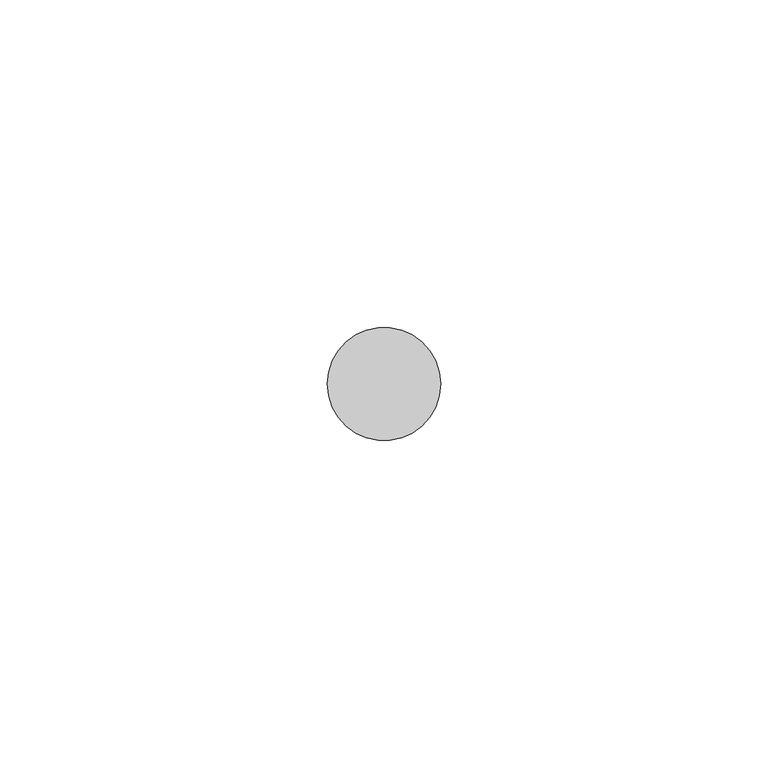
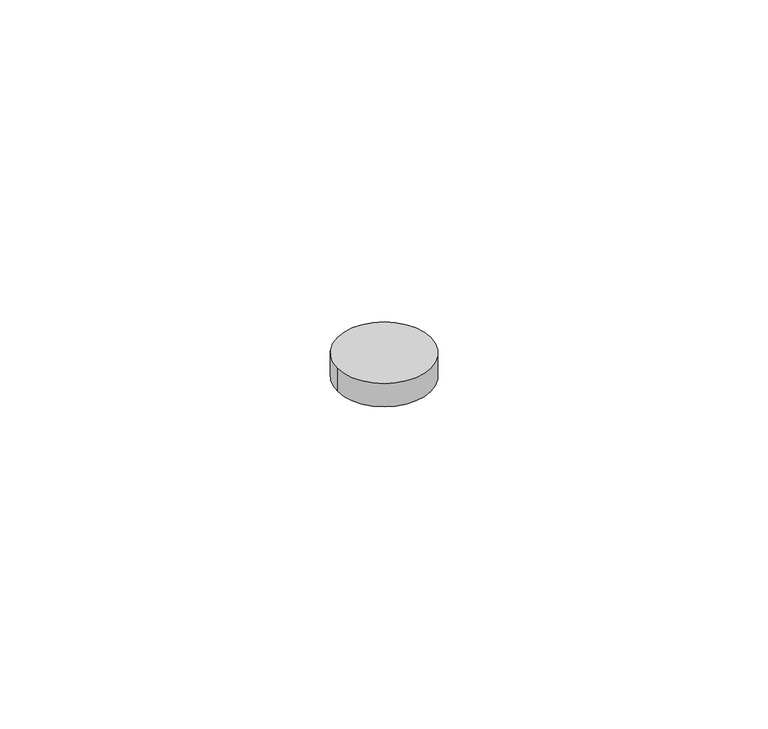
"""IFC4 building model written with IfcOpenShell, lengths in millimetres: proxy geometry, Hinge Pin Keeper14 : Hinge Pin Keeper."""

from ifc_helpers import new_model, si_unit, point, frame, frame_2d, origin, place, context, project, spatial, circle_curve, trimmed, segment, composite_curve, outline, extrude, source, transform, mapped, element, save


def generic_models_80a38197(model_context):
    return source(origin(), model_context, "Body", "SweptSolid", [
        extrude(outline(composite_curve([segment(trimmed(circle_curve(frame_2d((587319.1320739, -531776.6049841)), 8.6534625), [point((587310.4786114, -531776.6049841))], [point((587327.7855364, -531776.6049841))], False, "CARTESIAN"), True, "CONTINUOUS"), segment(trimmed(circle_curve(frame_2d((587319.1320739, -531776.6049841)), 8.6534625), [point((587327.7855364, -531776.6049841))], [point((587310.4786114, -531776.6049841))], False, "CARTESIAN"), True, "CONTINUOUS")], self_intersect=False)), frame((0.0, 0.0, 1271.7859375), z_axis=(0.0, 0.0, 1.0), x_axis=(1.0, 0.0, 0.0)), (0.0, 0.0, 1.0), 4.5640625),
    ])


if __name__ == "__main__":
    model = new_model("IFC4")
    model_context = context("Model", 3, world=origin())
    ifc_project = project(units=[si_unit("LENGTHUNIT", "METRE", prefix="MILLI")], contexts=[model_context])
    site = spatial("IfcSite", under=ifc_project)
    building = spatial("IfcBuilding", under=site)
    placement = place(None, origin())
    generic_models_shape = generic_models_80a38197(model_context)
    element("IfcBuildingElementProxy", 1, Name="Hinge Pin Keeper14 : Hinge Pin Keeper", ObjectType="Hinge Pin Keeper14 : Hinge Pin Keeper", at=placement, inside=building, context=model_context, shape_type="MappedRepresentation", body=[
        mapped(generic_models_shape, transform((0.0, 0.0, 0.0), x_axis=(1.0, 0.0, 0.0), y_axis=(0.0, 1.0, 0.0), z_axis=(0.0, 0.0, 1.0))),
    ])
    save(model, "model.ifc")

# Revit data of these elements
# Element 1 (IfcBuildingElementProxy, "Hinge Pin Keeper14 : Hinge Pin Keeper")
#   Materials on its faces: "6\"X6\" WELD-ON STL BUTT HINGE"
# Materials
#   "6\"X6\" WELD-ON STL BUTT HINGE": class "Metal", colour RGB 189 187 185, transparency 0, Description = "Carbon steel", Cost = 0
